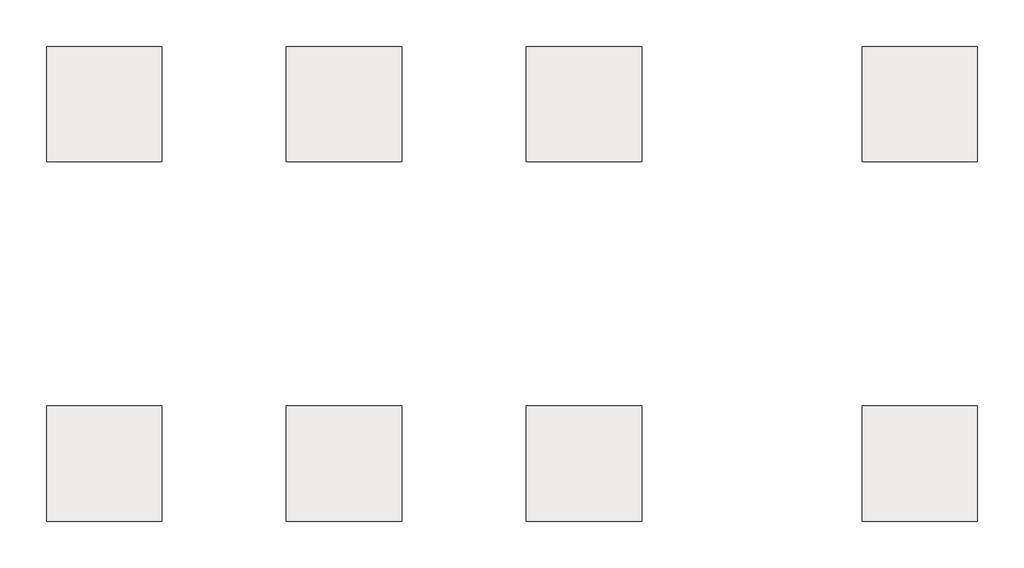
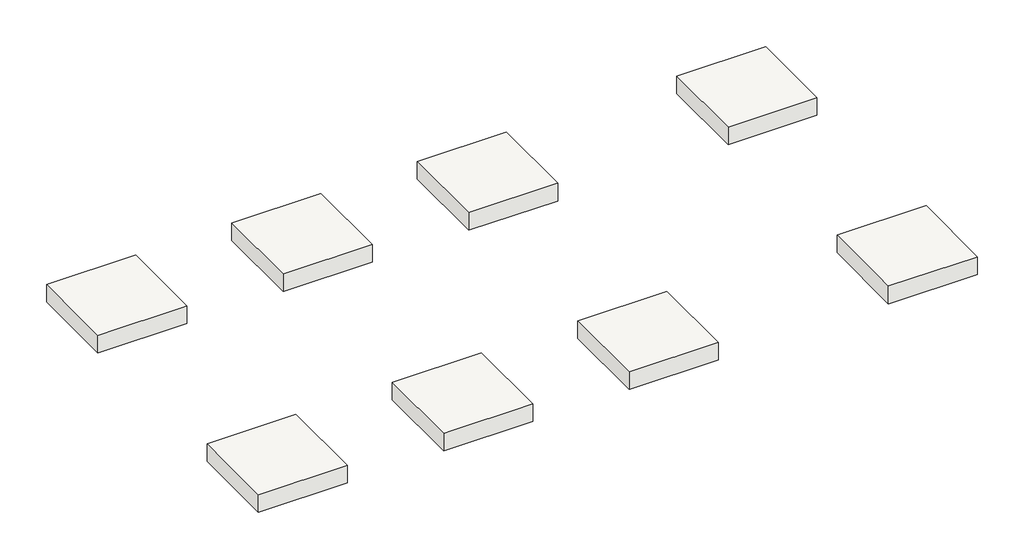
# Not in any storey: 8 slabs.
"""IFC4 building model written with IfcOpenShell, lengths in millimetres."""

import ifcopenshell
import ifcopenshell.guid

model = None  # the IFC model being written
_history = None  # IfcOwnerHistory: only IFC2X3 demands one
_inside = {}  # id of a spatial element -> (the spatial element, [elements in it])
_under = {}  # id of a project, library or spatial element -> (it, [spatial elements below it])
_declared = {}  # id of a project -> (the project, [libraries it declares])
_typed = {}  # id of a type object -> (the type object, [elements of that type])
_made_of = {}  # id of a material, layer set ... -> (it, [elements and type objects made of it])


def new_model(schema):
    """Start an empty IFC model of exactly this schema.

    Asked for "IFC4X3", IfcOpenShell would pick the latest addendum, in which some entities
    have other attributes; the version numbers below select the first issue.
    IFC2X3 requires an IfcOwnerHistory on every rooted entity: one is made here for all.
    """
    global model, _history
    if schema == "IFC4X3":
        model = ifcopenshell.file(schema_version=(4, 3, 0, 0))
    else:
        model = ifcopenshell.file(schema=schema)
    _inside.clear()
    _under.clear()
    _declared.clear()
    _typed.clear()
    _made_of.clear()
    _history = None
    if model.schema == "IFC2X3":
        org = make("IfcOrganization", Name="unknown")
        user = make(
            "IfcPersonAndOrganization",
            ThePerson=make("IfcPerson", FamilyName="unknown"),
            TheOrganization=org,
        )
        app = make(
            "IfcApplication",
            ApplicationDeveloper=org,
            Version="unknown",
            ApplicationFullName="unknown",
            ApplicationIdentifier="unknown",
        )
        _history = make(
            "IfcOwnerHistory",
            OwningUser=user,
            OwningApplication=app,
            ChangeAction="ADDED",
            CreationDate=0,
        )
    return model


def make(cls, **values):
    """One entity of the class cls with the attributes given. An attribute that is None is left unset."""
    return model.create_entity(
        cls, **{name: value for name, value in values.items() if value is not None}
    )


def rooted(cls, **values):
    """An entity with a GlobalId (a new one), such as an element, a storey or a relation."""
    return make(cls, GlobalId=ifcopenshell.guid.new(), OwnerHistory=_history, **values)


def si_unit(unit_type, name, prefix=None):
    """IfcSIUnit, for example si_unit("LENGTHUNIT", "METRE", prefix="MILLI")."""
    return make("IfcSIUnit", UnitType=unit_type, Prefix=prefix, Name=name)


def assignment(units):
    """IfcUnitAssignment: the units of a project."""
    return None if units is None else make("IfcUnitAssignment", Units=units)


def point(xyz):
    """IfcCartesianPoint."""
    return None if xyz is None else make("IfcCartesianPoint", Coordinates=xyz)


def direction(xyz):
    """IfcDirection."""
    return None if xyz is None else make("IfcDirection", DirectionRatios=xyz)


def frame(location, z_axis=None, x_axis=None):
    """IfcAxis2Placement3D, a coordinate frame: its origin and axes. An axis left out is left unset."""
    return make(
        "IfcAxis2Placement3D",
        Location=point(location),
        Axis=direction(z_axis),
        RefDirection=direction(x_axis),
    )


def origin():
    """The frame at (0, 0, 0) with its axes left unset."""
    return frame((0.0, 0.0, 0.0))


def place(relative_to, where):
    """IfcLocalPlacement: puts the frame where relative to a parent placement (None: the world)."""
    return make(
        "IfcLocalPlacement", PlacementRelTo=relative_to, RelativePlacement=where
    )


def context(
    kind, dimensions, precision=None, world=None, true_north=None, identifier=None
):
    """IfcGeometricRepresentationContext, for example the 3D "Model" context."""
    return make(
        "IfcGeometricRepresentationContext",
        ContextIdentifier=identifier,
        ContextType=kind,
        CoordinateSpaceDimension=dimensions,
        Precision=precision,
        WorldCoordinateSystem=world,
        TrueNorth=true_north,
    )


def project(units=None, contexts=None):
    """IfcProject with its units and contexts."""
    return rooted(
        "IfcProject",
        Name="project",
        RepresentationContexts=contexts,
        UnitsInContext=assignment(units),
    )


def spatial(cls, under=None, at=None, **own):
    """A site, building, storey or space (cls), placed at a placement, below another one or the project."""
    s = rooted(cls, ObjectPlacement=at, **own)
    if under is not None:
        _under.setdefault(under.id(), (under, []))[1].append(s)
    return s


def polyline(points):
    """IfcPolyline through the points."""
    return make("IfcPolyline", Points=[point(p) for p in points])


def outline(outer, holes=None, kind="AREA"):
    """IfcArbitraryClosedProfileDef: a profile drawn as a closed curve; with holes, ...WithVoids."""
    if holes is None:
        return make("IfcArbitraryClosedProfileDef", ProfileType=kind, OuterCurve=outer)
    return make(
        "IfcArbitraryProfileDefWithVoids",
        ProfileType=kind,
        OuterCurve=outer,
        InnerCurves=holes,
    )


def extrude(swept, where, along, depth):
    """IfcExtrudedAreaSolid: the profile swept, set in the frame where, extruded along a direction by depth."""
    return make(
        "IfcExtrudedAreaSolid",
        SweptArea=swept,
        Position=where,
        ExtrudedDirection=direction(along),
        Depth=depth,
    )


def shape(context_of_items, identifier, shape_type, items):
    """IfcShapeRepresentation: the items that make up one representation, for example the "Body"."""
    return make(
        "IfcShapeRepresentation",
        ContextOfItems=context_of_items,
        RepresentationIdentifier=identifier,
        RepresentationType=shape_type,
        Items=items,
    )


def source(mapping_origin, context_of_items, identifier, shape_type, items):
    """IfcRepresentationMap: a shape defined once, which mapped items show again and again."""
    return make(
        "IfcRepresentationMap",
        MappingOrigin=mapping_origin,
        MappedRepresentation=shape(context_of_items, identifier, shape_type, items),
    )


def transform(
    local_origin,
    x_axis=None,
    y_axis=None,
    z_axis=None,
    scale=None,
    scale2=None,
    scale3=None,
    uniform=True,
):
    """IfcCartesianTransformationOperator3D, or its non-uniform kind. x_axis, y_axis, z_axis: its Axis1, 2, 3."""
    if uniform:
        return make(
            "IfcCartesianTransformationOperator3D",
            Axis1=direction(x_axis),
            Axis2=direction(y_axis),
            LocalOrigin=point(local_origin),
            Scale=scale,
            Axis3=direction(z_axis),
        )
    return make(
        "IfcCartesianTransformationOperator3DnonUniform",
        Axis1=direction(x_axis),
        Axis2=direction(y_axis),
        LocalOrigin=point(local_origin),
        Scale=scale,
        Axis3=direction(z_axis),
        Scale2=scale2,
        Scale3=scale3,
    )


def mapped(mapping_source, mapping_target):
    """IfcMappedItem: shows the shape of a source again, moved by a transform."""
    return make(
        "IfcMappedItem", MappingSource=mapping_source, MappingTarget=mapping_target
    )


def made_of(thing, what):
    """Note that an element or type object is made of a material, layer set ...; save() writes the relation."""
    if what is not None:
        _made_of.setdefault(what.id(), (what, []))[1].append(thing)
    return thing


def element(
    cls,
    number,
    at=None,
    inside=None,
    cuts=None,
    type_object=None,
    material=None,
    context=None,
    identifier="Body",
    shape_type=None,
    held_by="IfcProductDefinitionShape",
    body=None,
    shapes=None,
    **own,
):
    """One element of the class cls, such as IfcWall. Its Tag is "e" and its number.

    at: its placement. inside: the storey or other place that contains it. cuts: it is an
    opening in that element (IfcRelVoidsElement). A single representation is given by context,
    identifier, shape_type and body (its items); several are given by shapes. held_by: the class
    of the entity that holds the representations. save() writes the other relations.
    """
    e = rooted(cls, Tag="e%d" % number, ObjectPlacement=at, **own)
    if body is not None:
        shapes = [shape(context, identifier, shape_type, body)]
    if shapes is not None:
        e.Representation = make(held_by, Representations=shapes)
    if inside is not None:
        _inside.setdefault(inside.id(), (inside, []))[1].append(e)
    if cuts is not None:
        rooted(
            "IfcRelVoidsElement", RelatingBuildingElement=cuts, RelatedOpeningElement=e
        )
    if type_object is not None:
        _typed.setdefault(type_object.id(), (type_object, []))[1].append(e)
    return made_of(e, material)


def aggregate(whole, parts):
    """IfcRelAggregates: a whole, such as a stair, and the parts it consists of."""
    return rooted("IfcRelAggregates", RelatingObject=whole, RelatedObjects=parts)


def save(model, path):
    """Write the relations noted so far, then the file.

    IfcRelAggregates (storeys below a building ...), IfcRelContainedInSpatialStructure (elements
    in a storey), IfcRelDefinesByType, IfcRelAssociatesMaterial and IfcRelDeclares: one each for
    every whole, place, type object, material and project.
    """
    for whole, parts in _under.values():
        aggregate(whole, parts)
    for where, things in _inside.values():
        rooted(
            "IfcRelContainedInSpatialStructure",
            RelatedElements=things,
            RelatingStructure=where,
        )
    for kind, things in _typed.values():
        rooted("IfcRelDefinesByType", RelatedObjects=things, RelatingType=kind)
    for what, things in _made_of.values():
        rooted("IfcRelAssociatesMaterial", RelatedObjects=things, RelatingMaterial=what)
    for by, libraries in _declared.values():
        rooted("IfcRelDeclares", RelatingContext=by, RelatedDefinitions=libraries)
    model.write(path)


def ft211_2400x2400x500_5fe39465(model_context):
    return source(origin(), model_context, "Body", "SweptSolid", [
        extrude(outline(polyline([(1200.0, 1200.0), (1200.0, -1200.0), (-1200.0, -1200.0), (-1200.0, 1200.0), (1200.0, 1200.0)])), frame((0.0, 0.0, -500.0), z_axis=(0.0, 0.0, 1.0), x_axis=(1.0, 0.0, 0.0)), (0.0, 0.0, 1.0), 500.0),
    ])


model = new_model("IFC4")

# Units and contexts
model_context = context("Model", 3, world=origin())
ifc_project = project(units=[si_unit("LENGTHUNIT", "METRE", prefix="MILLI")], contexts=[model_context])

# Site, building
site = spatial("IfcSite", under=ifc_project)
building = spatial("IfcBuilding", under=site)

# Slabs
placement = place(None, origin())
element("IfcSlab", 1, ObjectType="FT211-Footing-Rectangular_더미삭제 : FT211_2400x2400x500", at=placement, inside=building, context=model_context, shape_type="SweptSolid", body=[
    extrude(outline(polyline([(11200.0, 22199.5208589), (11200.0, 19799.5208589), (8800.0, 19799.5208589), (8800.0, 22199.5208589), (11200.0, 22199.5208589)])), frame((0.0, 0.0, -1800.0), z_axis=(0.0, 0.0, 1.0), x_axis=(1.0, 0.0, 0.0)), (0.0, 0.0, 1.0), 500.0),
])
element("IfcSlab", 2, ObjectType="FT211-Footing-Rectangular_더미삭제 : FT211_2400x2400x500", at=placement, inside=building, context=model_context, shape_type="SweptSolid", body=[
    extrude(outline(polyline([(6200.0, 22199.5208589), (6200.0, 19799.5208589), (3800.0, 19799.5208589), (3800.0, 22199.5208589), (6200.0, 22199.5208589)])), frame((0.0, 0.0, -1800.0), z_axis=(0.0, 0.0, 1.0), x_axis=(1.0, 0.0, 0.0)), (0.0, 0.0, 1.0), 500.0),
])
element("IfcSlab", 3, ObjectType="FT211-Footing-Rectangular_더미삭제 : FT211_2400x2400x500", at=placement, inside=building, context=model_context, shape_type="SweptSolid", body=[
    extrude(outline(polyline([(1200.0, 22199.5208589), (1200.0, 19799.5208589), (-1200.0, 19799.5208589), (-1200.0, 22199.5208589), (1200.0, 22199.5208589)])), frame((0.0, 0.0, -1800.0), z_axis=(0.0, 0.0, 1.0), x_axis=(1.0, 0.0, 0.0)), (0.0, 0.0, 1.0), 500.0),
])
element("IfcSlab", 4, ObjectType="FT211-Footing-Rectangular_더미삭제 : FT211_2400x2400x500", at=placement, inside=building, context=model_context, shape_type="SweptSolid", body=[
    extrude(outline(polyline([(1200.0, 14699.5208589), (1200.0, 12299.5208589), (-1200.0, 12299.5208589), (-1200.0, 14699.5208589), (1200.0, 14699.5208589)])), frame((0.0, 0.0, -1800.0), z_axis=(0.0, 0.0, 1.0), x_axis=(1.0, 0.0, 0.0)), (0.0, 0.0, 1.0), 500.0),
])
element("IfcSlab", 5, ObjectType="FT211-Footing-Rectangular_더미삭제 : FT211_2400x2400x500", at=placement, inside=building, context=model_context, shape_type="SweptSolid", body=[
    extrude(outline(polyline([(18200.0, 22199.5208589), (18200.0, 19799.5208589), (15800.0, 19799.5208589), (15800.0, 22199.5208589), (18200.0, 22199.5208589)])), frame((0.0, 0.0, -1800.0), z_axis=(0.0, 0.0, 1.0), x_axis=(1.0, 0.0, 0.0)), (0.0, 0.0, 1.0), 500.0),
])
ft211_2400x2400x500_shape = ft211_2400x2400x500_5fe39465(model_context)
element("IfcSlab", 6, ObjectType="FT211-Footing-Rectangular_더미삭제 : FT211_2400x2400x500", at=placement, inside=building, context=model_context, shape_type="MappedRepresentation", body=[
    mapped(ft211_2400x2400x500_shape, transform((5000.0, 13499.5208589, -1300.0), x_axis=(1.0, 0.0, 0.0), y_axis=(0.0, 1.0, 0.0), z_axis=(0.0, 0.0, 1.0))),
])
element("IfcSlab", 7, ObjectType="FT211-Footing-Rectangular_더미삭제 : FT211_2400x2400x500", at=placement, inside=building, context=model_context, shape_type="MappedRepresentation", body=[
    mapped(ft211_2400x2400x500_shape, transform((10000.0, 13499.5208589, -1300.0), x_axis=(1.0, 0.0, 0.0), y_axis=(0.0, 1.0, 0.0), z_axis=(0.0, 0.0, 1.0))),
])
element("IfcSlab", 8, ObjectType="FT211-Footing-Rectangular_더미삭제 : FT211_2400x2400x500", at=placement, inside=building, context=model_context, shape_type="MappedRepresentation", body=[
    mapped(ft211_2400x2400x500_shape, transform((17000.0, 13499.5208589, -1300.0), x_axis=(1.0, 0.0, 0.0), y_axis=(0.0, 1.0, 0.0), z_axis=(0.0, 0.0, 1.0))),
])

save(model, "model.ifc")

# Revit data of these elements
# Project information
#   Building Name = "MAIN GATE SECURITY BUILDING"
#   Project Status = "Project Status"
#   Client Name = "현대엔지니어링"
#   Project Address = "서울시 종로구 율곡로 75(계동)"
#   Project Name = "Therma Visayas Energy Project"
#   Project Number = "-"
# Grids (mm)
#   "A": line (0, 24502.793) -> (0, 11308.625)
#   "B": line (5000, 24502.793) -> (5000, 11308.625)
#   "C": line (10000, 24502.793) -> (10000, 11308.625)
#   "1": line (-3860.098, 13499.521) -> (12441.468, 13499.521)
#   "2": line (-3860.098, 20999.521) -> (12441.468, 20999.521)
# Type "FT211-Footing-Rectangular_더미삭제 : FT211_2400x2400x500"
#   Top bar = "D25@300"
#   Description = "UG Shallow Foundation"
#   Bottom bar = "D20@300"
#   Width = 2400 mm
#   Length = 2400 mm
#   Foundation Thickness = 500 mm
#   Structural Material [instance default] = A03AC032-00007_Structural Concrete_Type1_25MPa-30Mpa
#   Assembly Code = ""
# Elements 1, 2, 3, 4, 6, 7 (IfcSlab, "FT211-Footing-Rectangular_더미삭제 : FT211_2400x2400x500")
#   Comments = ""
#   Mark = "F1"
#   F01) Building Name = "Main Gate House"
#   F11) Project Building Tag_Type-1 = "Common"
#   F12) Project Building Tag_Type-2 = "Common"
#   F13) Project Facility Code = "Facility Code"
#   F21) Structural Type = "Concrete"
#   F31) Standard Building Code = "IBC"
#   F41) Discipline = "AR"
#   F51) Plan Start Date-Engineering = "2015-01-01"
#   F52) Plan Finish Date-Engineering = "2015-12-31"
#   F53) Duration = "365"
#   F54) Actual Start Date-Engineering = "2015-01-01"
#   F55) Actual Finish Date-Engineering = "2015-12-31"
#   F61) Plan Start Date-Construction = "2016-08-19"
#   F62) Plan Finish Date-Construction = "2017-01-31"
#   F64) Actual Start Date-Construction = "2016-08-19"
#   F63) Duration = "202"
#   F65) Actual Finish Date-Construction = "2017-01-31"
#   F91) Plant Type = "CFPP"
#   F92) KKS Structures, Building = "UYF"
#   P01) Project Name = "TVEP"
#   P02) Project Configuration = "CFB Boiler x 2(Foster Wheeler) + STG x 2(Alstom, 150MW)"
#   P03) Project Abbreviation = "TVEP"
#   P04) Project Code = "BEPH1402"
#   P05) Project Stage = "In operation"
#   P06) Project Location = "Sito Looc, Barangay Bato, Toledo City in Philippines"
#   P07) Project Owner = "Therma Visayas, Inc."
#   P08) Project O.E = "Flour"
#   P09) Project Schedule = "ITB Issueing Date : 2013.07.30\r\nSite Survey : 2013.08.19-20\r\nBid Closing Date : 2013.11.29\r\nPreferred Bidder Notice 접수 : 2014.04.27\r\nTarget award date : 2014 05\r\nLOA 접수 : 2014.05.21\r\nSigning Ceremony : 2014.05.30"
#   P10) Basic Wind Speed = "55.6 m/s"
#   P11) Seismic = "NSCP 2010, Zone 4 (PGA : 0.4g)"
#   P12) Soil = "Sc"
#   P13) Soil Capacity = "100kN/m2"
#   P14) Pile Capacity = "PHC(D400) : 1200kN"
#   W00) Work Master Code = "A03AC032-00007"
#   W01) Work Master_Lv1 = "Concrete Work"
#   W02) Work Master_Lv2 = "Substructure Work"
#   W03) Work Master_Spec.1 = "Cement Type-1"
#   W04) Work Master_Spec.2 = "25MPa < F'c (Cylinder Strength) ≤ 30MPa"
#   W11) Activity ID = "C02AGB010"
#   W12) Activity Name = "Main Gate Security Building - Building Foundation"
#   W13) Plan Start Date = "2016-08-19"
#   W14) Plan Finish Date = "2016-09-22"
#   W15) Duration = "26"
#   W16) Actual Start Date = "2016-08-19"
#   W17) Actual Finish Date = "2016-09-22"
#   R02) Unit Price = 0
#   Structural Material = A03AC032-00007_Structural Concrete_Type1_25MPa-30Mpa
#   Phase Created = New Construction
#   Materials on its faces: "A03AC032-00007_Structural Concrete_Type1_25MPa-30Mpa"
# Elements 5, 8 (IfcSlab, "FT211-Footing-Rectangular_더미삭제 : FT211_2400x2400x500")
#   Comments = ""
#   F01) Building Name = "Main Gate House"
#   F11) Project Building Tag_Type-1 = "Common"
#   F12) Project Building Tag_Type-2 = "Common"
#   F13) Project Facility Code = "Facility Code"
#   F21) Structural Type = "Concrete"
#   F31) Standard Building Code = "IBC"
#   F41) Discipline = "AR"
#   F51) Plan Start Date-Engineering = "2015-01-01"
#   F52) Plan Finish Date-Engineering = "2015-12-31"
#   F53) Duration = "365"
#   F54) Actual Start Date-Engineering = "2015-01-01"
#   F55) Actual Finish Date-Engineering = "2015-12-31"
#   F61) Plan Start Date-Construction = "2016-08-19"
#   F62) Plan Finish Date-Construction = "2017-01-31"
#   F64) Actual Start Date-Construction = "2016-08-19"
#   F63) Duration = "202"
#   F65) Actual Finish Date-Construction = "2017-01-31"
#   F91) Plant Type = "CFPP"
#   F92) KKS Structures, Building = "UYF"
#   P01) Project Name = "TVEP"
#   P02) Project Configuration = "CFB Boiler x 2(Foster Wheeler) + STG x 2(Alstom, 150MW)"
#   P03) Project Abbreviation = "TVEP"
#   P04) Project Code = "BEPH1402"
#   P05) Project Stage = "In operation"
#   P06) Project Location = "Sito Looc, Barangay Bato, Toledo City in Philippines"
#   P07) Project Owner = "Therma Visayas, Inc."
#   P08) Project O.E = "Flour"
#   P09) Project Schedule = "ITB Issueing Date : 2013.07.30\r\nSite Survey : 2013.08.19-20\r\nBid Closing Date : 2013.11.29\r\nPreferred Bidder Notice 접수 : 2014.04.27\r\nTarget award date : 2014 05\r\nLOA 접수 : 2014.05.21\r\nSigning Ceremony : 2014.05.30"
#   P10) Basic Wind Speed = "55.6 m/s"
#   P11) Seismic = "NSCP 2010, Zone 4 (PGA : 0.4g)"
#   P12) Soil = "Sc"
#   P13) Soil Capacity = "100kN/m2"
#   P14) Pile Capacity = "PHC(D400) : 1200kN"
#   W00) Work Master Code = "A03AC032-00007"
#   W01) Work Master_Lv1 = "Concrete Work"
#   W02) Work Master_Lv2 = "Substructure Work"
#   W03) Work Master_Spec.1 = "Cement Type-1"
#   W04) Work Master_Spec.2 = "25MPa < F'c (Cylinder Strength) ≤ 30MPa"
#   W11) Activity ID = "C02AGB010"
#   W12) Activity Name = "Main Gate Security Building - Building Foundation"
#   W13) Plan Start Date = "2016-08-19"
#   W14) Plan Finish Date = "2016-09-22"
#   W15) Duration = "26"
#   W16) Actual Start Date = "2016-08-19"
#   W17) Actual Finish Date = "2016-09-22"
#   R02) Unit Price = 0
#   Structural Material = A03AC032-00007_Structural Concrete_Type1_25MPa-30Mpa
#   Phase Created = New Construction
#   Materials on its faces: "A03AC032-00007_Structural Concrete_Type1_25MPa-30Mpa"
# Materials
#   "A03AC032-00007_Structural Concrete_Type1_25MPa-30Mpa": class "Concrete", colour RGB 176 176 176, transparency 0, Keynote = "09910.A1", Description = "Reinf. Conc.", W00) Work Master Code = "A03AC032-00007", W01) Work Master_Lv1 = "Concrete Work", W02) Work Master_Lv2 = "Substructure Work", W03) Work Master_Spec.1 = "Structural Concrete", W04) Work Master_Spec.2 = "Cement Type-1", W05) Work Master_Spec.3 = "25MPa < F'c (Cylinder Strength) ≤ 30MPa", Cost = 0
